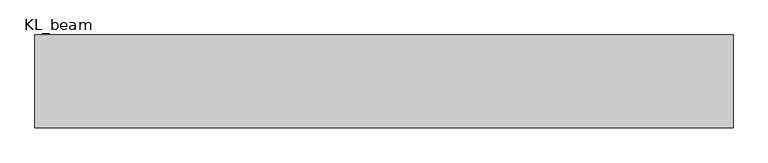
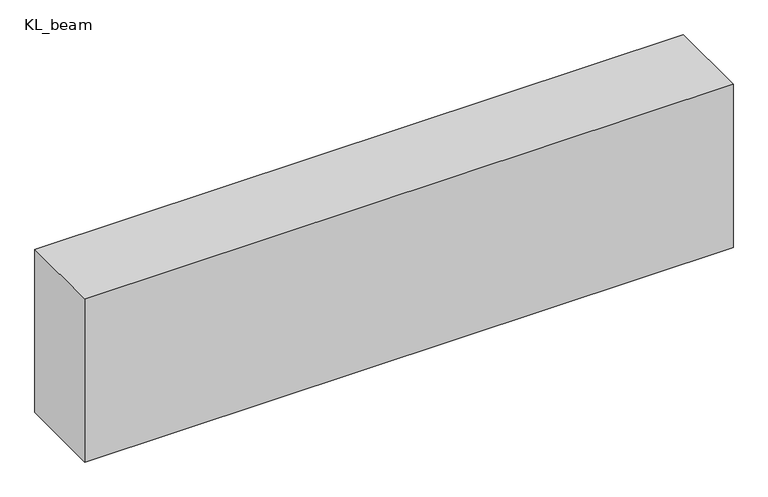
"""IFC4 building model written with IfcOpenShell, lengths in millimetres: beam geometry, 混凝土 - 矩形梁 : KL_beam."""

from ifc_helpers import new_model, si_unit, frame, origin, place, context, project, spatial, polyline, outline, extrude, source, transform, mapped, element, save


def kl_beam_7cc9d33b(model_context):
    return source(origin(), model_context, "Body", "SweptSolid", [
        extrude(outline(polyline([(1501.5, 200.0), (1501.5, -200.0), (-1501.5, -200.0), (-1501.5, 200.0), (1501.5, 200.0)])), frame((0.0, 0.0, -400.0), z_axis=(0.0, 0.0, 1.0), x_axis=(1.0, 0.0, 0.0)), (0.0, 0.0, 1.0), 800.0),
    ])


if __name__ == "__main__":
    model = new_model("IFC4")
    model_context = context("Model", 3, world=origin())
    ifc_project = project(units=[si_unit("LENGTHUNIT", "METRE", prefix="MILLI")], contexts=[model_context])
    site = spatial("IfcSite", under=ifc_project)
    building = spatial("IfcBuilding", under=site)
    placement = place(None, origin())
    kl_beam_shape = kl_beam_7cc9d33b(model_context)
    element("IfcBeam", 1, ObjectType="混凝土 - 矩形梁 : KL_beam", at=placement, inside=building, context=model_context, shape_type="MappedRepresentation", body=[
        mapped(kl_beam_shape, transform((0.0, 0.0, 0.0), x_axis=(1.0, 0.0, 0.0), y_axis=(0.0, 1.0, 0.0), z_axis=(0.0, 0.0, 1.0))),
    ])
    save(model, "model.ifc")

# Revit data of these elements
# Type "混凝土 - 矩形梁 : KL_beam"
#   Length [instance default] = 1524 mm
#   b = 400 mm
#   h = 800 mm
#   Structural Material [instance default] = 混凝土 - 现场浇注混凝土
#   Assembly Code = ""
# Element 1 (IfcBeam, "混凝土 - 矩形梁 : KL_beam")
#   Structural Material = none
# Materials
#   "混凝土 - 现场浇注混凝土": class "混凝土", colour RGB 192 192 192, transparency 0
